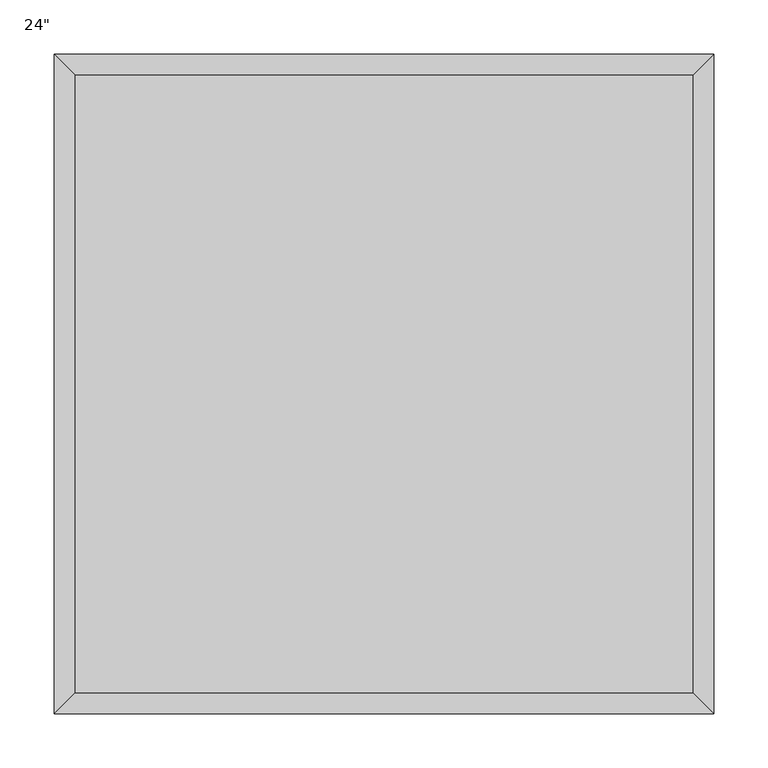
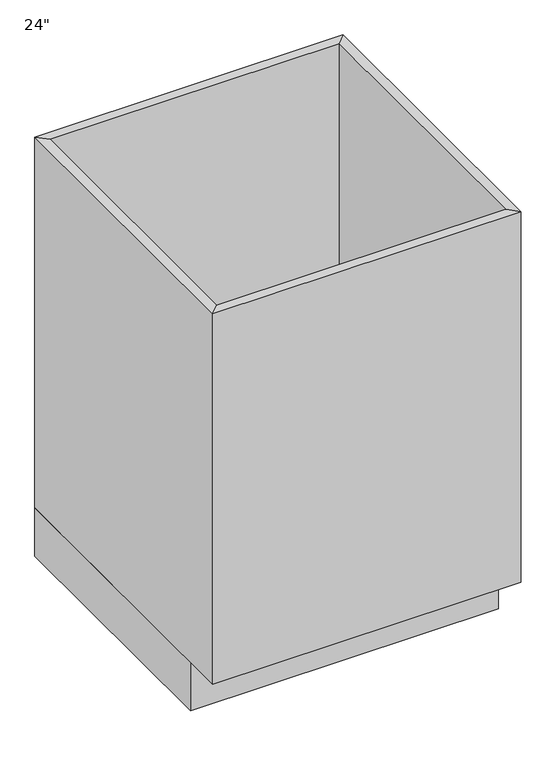
"""IFC4 building model written with IfcOpenShell, lengths in millimetres: furniture geometry."""

from ifc_helpers import new_model, si_unit, frame, origin, origin_with_axes, place, context, project, spatial, polyline, outline, extrude, faceted_brep, source, transform, mapped, element, save


def furniture_ee806227(model_context):
    return source(origin(), model_context, "Body", "SolidModel", [
        extrude(outline(polyline([(304.4877049, -19.05), (304.4877049, -590.55), (-267.0122951, -590.55), (-267.0122951, -19.05), (304.4877049, -19.05)])), frame((0.0, 0.0, 101.6), z_axis=(0.0, 0.0, 1.0), x_axis=(1.0, 0.0, 0.0)), (0.0, 0.0, 1.0), 19.05),
        faceted_brep([(304.4877049, -590.55, 876.3), (304.4877049, -590.55, 101.6), (-267.0122951, -590.55, 101.6), (-267.0122951, -590.55, 876.3), (323.5377049, -609.6, 876.3), (-286.0622951, -609.6, 876.3), (323.5377049, -609.6, 101.6), (-286.0622951, -609.6, 101.6), (-267.0122951, -19.05, 101.6), (-267.0122951, -19.05, 876.3), (-286.0622951, 0.0, 876.3), (-286.0622951, 0.0, 101.6), (304.4877049, -19.05, 101.6), (304.4877049, -19.05, 876.3), (323.5377049, 0.0, 876.3), (323.5377049, 0.0, 101.6)], [[[0, 1, 2, 3]], [[4, 0, 3, 5]], [[6, 4, 5, 7]], [[1, 6, 7, 2]], [[3, 2, 8, 9]], [[5, 3, 9, 10]], [[7, 5, 10, 11]], [[2, 7, 11, 8]], [[9, 8, 12, 13]], [[10, 9, 13, 14]], [[11, 10, 14, 15]], [[8, 11, 15, 12]], [[13, 12, 1, 0]], [[14, 13, 0, 4]], [[15, 14, 4, 6]], [[12, 15, 6, 1]]]),
        extrude(outline(polyline([(323.5377049, 0.0), (323.5377049, -533.4), (-286.0622951, -533.4), (-286.0622951, 0.0), (323.5377049, 0.0)])), origin_with_axes(), (0.0, 0.0, 1.0), 101.6),
    ])


if __name__ == "__main__":
    model = new_model("IFC4")
    model_context = context("Model", 3, world=origin())
    ifc_project = project(units=[si_unit("LENGTHUNIT", "METRE", prefix="MILLI")], contexts=[model_context])
    site = spatial("IfcSite", under=ifc_project)
    building = spatial("IfcBuilding", under=site)
    placement = place(None, origin())
    furniture_shape = furniture_ee806227(model_context)
    element("IfcFurniture", 1, ObjectType="Base Cabinet-Single Door & Drawer : 24\"", at=placement, inside=building, context=model_context, shape_type="MappedRepresentation", body=[
        mapped(furniture_shape, transform((0.0, 0.0, 0.0), x_axis=(1.0, 0.0, 0.0), y_axis=(0.0, 1.0, 0.0), z_axis=(0.0, 0.0, 1.0))),
    ])
    save(model, "model.ifc")

# Revit data of these elements
# Type "Base Cabinet-Single Door & Drawer : 24\""
#   Depth = 2' - 0"
#   Height = 2' - 10 1/2"
#   Toe Depth = 0' - 3"
#   Toe Height = 0' - 4"
#   Width = 2' - 0"
# Element 1 (IfcFurniture, "Base Cabinet-Single Door & Drawer : 24\"")
#   Materials on its faces: "Cabinet"
# Materials
#   "Cabinet": class "Wood", colour RGB 189 170 130, transparency 0, Cost = 0
